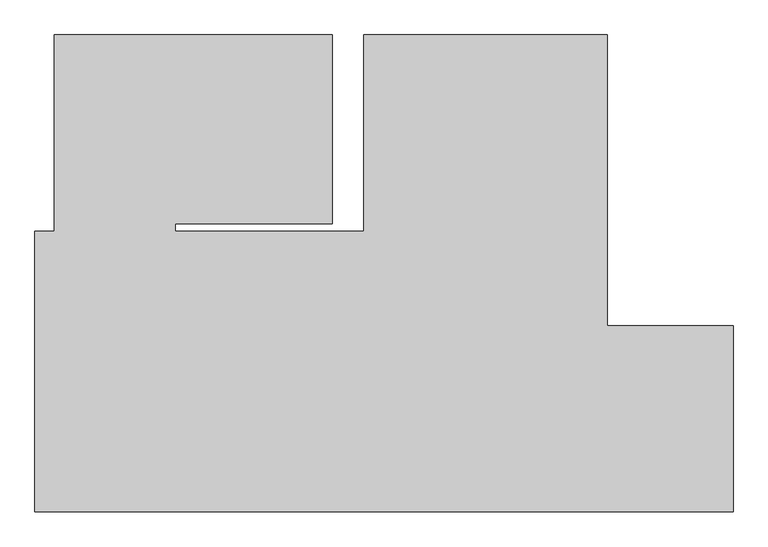
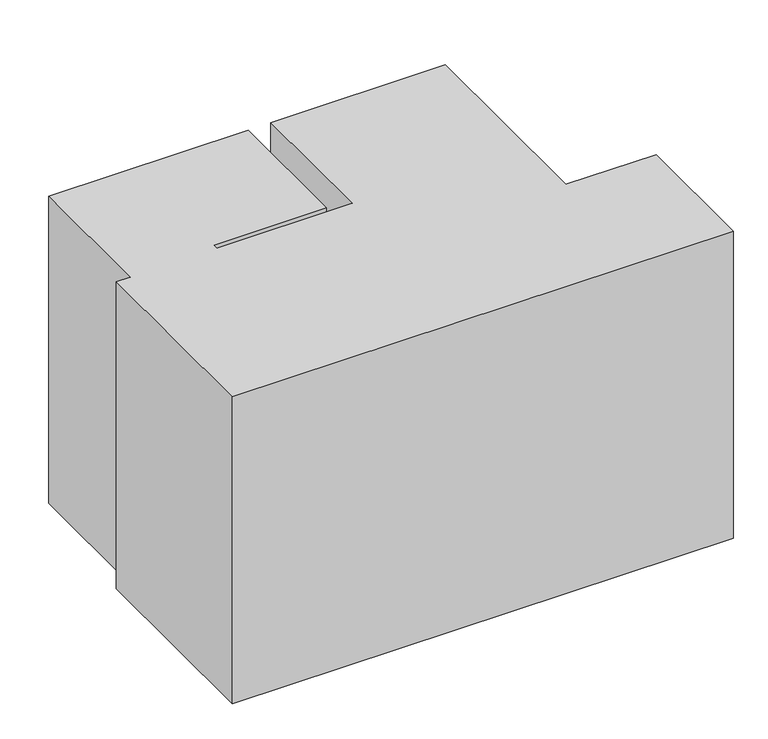
"""IFC4 building model written with IfcOpenShell, lengths in millimetres: proxy geometry, 0_3d."""

from ifc_helpers import new_model, si_unit, origin, origin_with_axes, place, context, project, spatial, polyline, outline, extrude, source, transform, mapped, element, save


def generic_models_528b9666(model_context):
    return source(origin(), model_context, "Body", "SweptSolid", [
        extrude(outline(polyline([(122.0, 1783.4), (122.0, 3033.3404327), (1892.0000064, 3033.3404327), (1892.0000064, 1833.3404327), (892.0000064, 1833.3404327), (892.0000064, 1783.3404327), (2092.0000064, 1783.3404327), (2092.0000064, 3033.3404394), (3642.0000032, 3033.4), (3642.1609942, 1233.4000072), (3642.1609938, 1183.4000072), (4442.0, 1183.4), (4442.0, 0.0), (0.0, 0.0), (0.0, 1783.4), (122.0, 1783.4)])), origin_with_axes(), (0.0, 0.0, 1.0), 2880.0),
    ])


if __name__ == "__main__":
    model = new_model("IFC4")
    model_context = context("Model", 3, world=origin())
    ifc_project = project(units=[si_unit("LENGTHUNIT", "METRE", prefix="MILLI")], contexts=[model_context])
    site = spatial("IfcSite", under=ifc_project)
    building = spatial("IfcBuilding", under=site)
    placement = place(None, origin())
    generic_models_shape = generic_models_528b9666(model_context)
    element("IfcBuildingElementProxy", 1, Name="0_3d", ObjectType="0_3d", at=placement, inside=building, context=model_context, shape_type="MappedRepresentation", body=[
        mapped(generic_models_shape, transform((0.0, 0.0, 0.0), x_axis=(1.0, 0.0, 0.0), y_axis=(0.0, 1.0, 0.0), z_axis=(0.0, 0.0, 1.0))),
    ])
    save(model, "model.ifc")

# Revit data of these elements
# Element 1 (IfcBuildingElementProxy, "0_3d")
#   Materials on its faces: "*1"
# Materials
#   "*1": class "Unassigned", colour RGB 175 175 175, transparency 0
